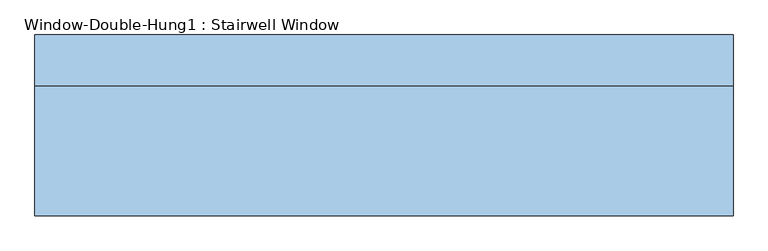
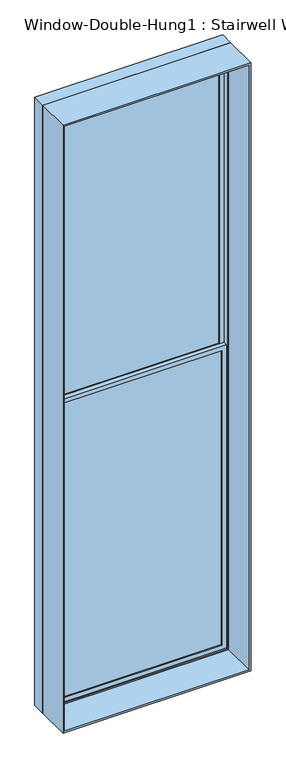
"""IFC4 building model written with IfcOpenShell, lengths in millimetres: window geometry, Window-Double-Hung1 : Stairwell Window."""

from ifc_helpers import new_model, si_unit, frame, origin, place, context, project, spatial, polyline, outline, extrude, source, transform, mapped, element, save


def window_double_hung1_stairwell_window_f29d4600(model_context):
    return source(origin(), model_context, "Body", "SweptSolid", [
        extrude(outline(polyline([(838.2, 157.1625), (838.2, 150.8125), (-838.2, 150.8125), (-838.2, 157.1625), (838.2, 157.1625)])), frame((0.0, 0.0, 990.6), z_axis=(0.0, 0.0, 1.0), x_axis=(1.0, 0.0, 0.0)), (0.0, 0.0, 1.0), 3025.775),
        extrude(outline(polyline([(-838.2, 144.4625), (838.2, 144.4625), (838.2, 138.1125), (-838.2, 138.1125), (-838.2, 144.4625)])), frame((0.0, 0.0, 990.6), z_axis=(0.0, 0.0, 1.0), x_axis=(1.0, 0.0, 0.0)), (0.0, 0.0, 1.0), 3025.775),
        extrude(outline(polyline([(838.2, 201.6125), (838.2, 195.2625), (-838.2, 195.2625), (-838.2, 201.6125), (838.2, 201.6125)])), frame((0.0, 0.0, 4060.825), z_axis=(0.0, 0.0, 1.0), x_axis=(1.0, 0.0, 0.0)), (0.0, 0.0, 1.0), 3025.775),
        extrude(outline(polyline([(-838.2, 188.9125), (838.2, 188.9125), (838.2, 182.5625), (-838.2, 182.5625), (-838.2, 188.9125)])), frame((0.0, 0.0, 4060.825), z_axis=(0.0, 0.0, 1.0), x_axis=(1.0, 0.0, 0.0)), (0.0, 0.0, 1.0), 3025.775),
        extrude(outline(polyline([(4060.825, -882.65), (946.15, -882.65), (946.15, 882.65), (4060.825, 882.65), (4060.825, -882.65)]), holes=[polyline([(4016.375, 838.2), (990.6, 838.2), (990.6, -838.2), (4016.375, -838.2), (4016.375, 838.2)])]), frame((0.0, 125.4125, 0.0), z_axis=(0.0, 1.0, 0.0), x_axis=(0.0, 0.0, 1.0)), (0.0, 0.0, 1.0), 44.45),
        extrude(outline(polyline([(7131.05, -882.65), (4016.375, -882.65), (4016.375, 882.65), (7131.05, 882.65), (7131.05, -882.65)]), holes=[polyline([(7086.6, 838.2), (4060.825, 838.2), (4060.825, -838.2), (7086.6, -838.2), (7086.6, 838.2)])]), frame((0.0, 169.8625, 0.0), z_axis=(0.0, 1.0, 0.0), x_axis=(0.0, 0.0, 1.0)), (0.0, 0.0, 1.0), 44.45),
        extrude(outline(polyline([(7162.8, -914.4), (914.4, -914.4), (914.4, 914.4), (7162.8, 914.4), (7162.8, -914.4)]), holes=[polyline([(7131.05, 882.65), (946.15, 882.65), (946.15, -882.65), (7131.05, -882.65), (7131.05, 882.65)])]), frame((0.0, 112.7125, 0.0), z_axis=(0.0, 1.0, 0.0), x_axis=(0.0, 0.0, 1.0)), (0.0, 0.0, 1.0), 133.35),
        extrude(outline(polyline([(7162.8, 914.4), (7162.8, -914.4), (914.4, -914.4), (914.4, 914.4), (7162.8, 914.4)]), holes=[polyline([(7143.75, 895.35), (933.45, 895.35), (933.45, -895.35), (7143.75, -895.35), (7143.75, 895.35)])]), frame((0.0, -227.0125, 0.0), z_axis=(0.0, 1.0, 0.0), x_axis=(0.0, 0.0, 1.0)), (0.0, 0.0, 1.0), 339.725),
    ])


if __name__ == "__main__":
    model = new_model("IFC4")
    model_context = context("Model", 3, world=origin())
    ifc_project = project(units=[si_unit("LENGTHUNIT", "METRE", prefix="MILLI")], contexts=[model_context])
    site = spatial("IfcSite", under=ifc_project)
    building = spatial("IfcBuilding", under=site)
    placement = place(None, origin())
    window_double_hung1_stairwell_window_shape = window_double_hung1_stairwell_window_f29d4600(model_context)
    element("IfcWindow", 1, ObjectType="Window-Double-Hung1 : Stairwell Window", at=placement, inside=building, context=model_context, shape_type="MappedRepresentation", body=[
        mapped(window_double_hung1_stairwell_window_shape, transform((0.0, 0.0, 0.0), x_axis=(1.0, 0.0, 0.0), y_axis=(0.0, 1.0, 0.0), z_axis=(0.0, 0.0, 1.0))),
    ])
    save(model, "model.ifc")

# Revit data of these elements
# Type "Window-Double-Hung1 : Stairwell Window"
#   Type Mark = "WT-13"
#   Fire Rating = "0.5h"
#   Construction Type Id = "DG-DR"
#   Assembly Code = "B2020100"
#   Analytic Construction = "Double glazing - domestic"
#   Wall Thickness [instance default] = 0' - 6"
#   Window Inset [instance default] = 0' - 0"
#   Visual Light Transmittance = 0.81
#   Thermal Resistance (R) = 1.8146 (h·ft²·°F)/BTU
#   Solar Heat Gain Coefficient = 0.76
#   Muntin Width = 5' - 6"
#   Muntin Height = 9' - 11 1/8"
#   Interior Wall Closure [instance default] = 0' - 1 1/2"
#   Rough Width = 6' - 0 1/2"
#   Rough Height = 20' - 6 1/2"
#   Frame Extension [instance default] = 0' - 1 1/4"
#   Exterior Wall Closure [instance default] = 0' - 0 1/2"
#   Extension Jamb [instance default] = 0' - 1 1/2"
#   Heat Transfer Coefficient (U) = 0.5511 BTU/(h·ft²·°F)
#   Height = 20' - 6"
#   Width = 6' - 0"
#   Top Muntin Visibility = no
#   Indicator Visibility [instance default] = yes
#   Extension Jamb Visibility [instance default] = yes
#   Interior Trim Visibility [instance default] = yes
#   Exterior Trim Visibility [instance default] = yes
#   Define Thermal Properties by = 1
#   Bottom Muntin Visibility = no
#   Muntin Pattern = Trim-Window-Exterior-Flat : with Sill
#   Interior Trim Material = Wood - Stained
#   Interior Trim = Trim-Window-Interior-Flat : Picture Frame
#   Exterior Trim Material = Clad - White
#   Exterior Trim = Trim-Window-Exterior-Flat : with Sill
#   Glass Panel Material = Glass
#   Exterior Frame Material = Clad - White
#   Interior Frame Material = Wood - Stained
#   Wall Closure = (empty or 0)
# Element 1 (IfcWindow, "Window-Double-Hung1 : Stairwell Window")
#   Wall Thickness = 1' - 5 7/8"
#   Extension Jamb = 1' - 1 3/8"
#   Materials on its faces: "Wood - Stained", "Glass", "Clad - White"
# Materials
#   "Wood - Stained": class "Wood", colour RGB 224 178 126, transparency 0, Cost = 0
#   "Clad - White": class "Wood", colour RGB 242 242 238, transparency 0, Cost = 0
#   "Glass": class "Glass", colour RGB 0 128 192, transparency 0.75, Description = "Soda Lime Glass", Cost = 0
